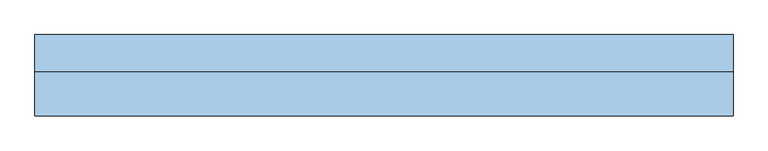
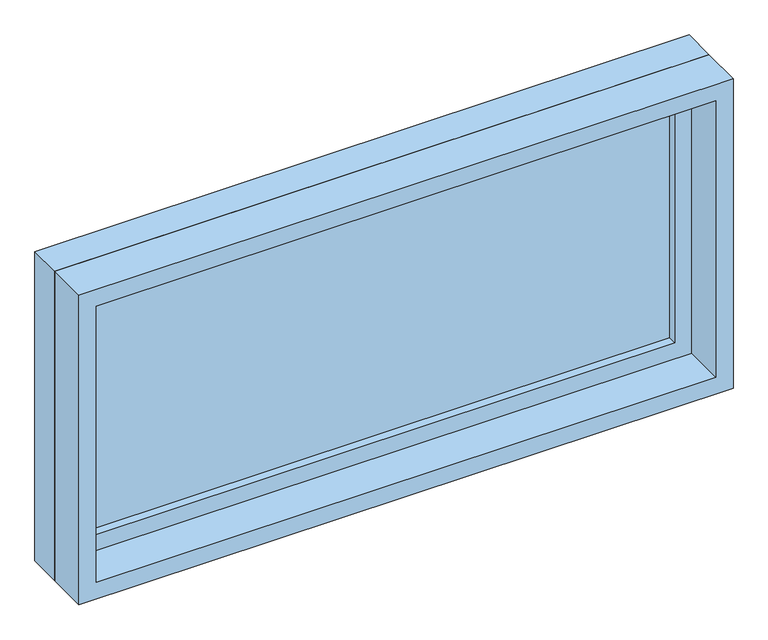
"""IFC4 building model written with IfcOpenShell, lengths in millimetres: window geometry, Фиксированные : 1200х600."""

import ifcopenshell
import ifcopenshell.guid

model = None  # the IFC model being written
_history = None  # IfcOwnerHistory: only IFC2X3 demands one
_inside = {}  # id of a spatial element -> (the spatial element, [elements in it])
_under = {}  # id of a project, library or spatial element -> (it, [spatial elements below it])
_declared = {}  # id of a project -> (the project, [libraries it declares])
_typed = {}  # id of a type object -> (the type object, [elements of that type])
_made_of = {}  # id of a material, layer set ... -> (it, [elements and type objects made of it])


def new_model(schema):
    """Start an empty IFC model of exactly this schema.

    Asked for "IFC4X3", IfcOpenShell would pick the latest addendum, in which some entities
    have other attributes; the version numbers below select the first issue.
    IFC2X3 requires an IfcOwnerHistory on every rooted entity: one is made here for all.
    """
    global model, _history
    if schema == "IFC4X3":
        model = ifcopenshell.file(schema_version=(4, 3, 0, 0))
    else:
        model = ifcopenshell.file(schema=schema)
    _inside.clear()
    _under.clear()
    _declared.clear()
    _typed.clear()
    _made_of.clear()
    _history = None
    if model.schema == "IFC2X3":
        org = make("IfcOrganization", Name="unknown")
        user = make(
            "IfcPersonAndOrganization",
            ThePerson=make("IfcPerson", FamilyName="unknown"),
            TheOrganization=org,
        )
        app = make(
            "IfcApplication",
            ApplicationDeveloper=org,
            Version="unknown",
            ApplicationFullName="unknown",
            ApplicationIdentifier="unknown",
        )
        _history = make(
            "IfcOwnerHistory",
            OwningUser=user,
            OwningApplication=app,
            ChangeAction="ADDED",
            CreationDate=0,
        )
    return model


def make(cls, **values):
    """One entity of the class cls with the attributes given. An attribute that is None is left unset."""
    return model.create_entity(
        cls, **{name: value for name, value in values.items() if value is not None}
    )


def rooted(cls, **values):
    """An entity with a GlobalId (a new one), such as an element, a storey or a relation."""
    return make(cls, GlobalId=ifcopenshell.guid.new(), OwnerHistory=_history, **values)


def si_unit(unit_type, name, prefix=None):
    """IfcSIUnit, for example si_unit("LENGTHUNIT", "METRE", prefix="MILLI")."""
    return make("IfcSIUnit", UnitType=unit_type, Prefix=prefix, Name=name)


def assignment(units):
    """IfcUnitAssignment: the units of a project."""
    return None if units is None else make("IfcUnitAssignment", Units=units)


def point(xyz):
    """IfcCartesianPoint."""
    return None if xyz is None else make("IfcCartesianPoint", Coordinates=xyz)


def direction(xyz):
    """IfcDirection."""
    return None if xyz is None else make("IfcDirection", DirectionRatios=xyz)


def frame(location, z_axis=None, x_axis=None):
    """IfcAxis2Placement3D, a coordinate frame: its origin and axes. An axis left out is left unset."""
    return make(
        "IfcAxis2Placement3D",
        Location=point(location),
        Axis=direction(z_axis),
        RefDirection=direction(x_axis),
    )


def origin():
    """The frame at (0, 0, 0) with its axes left unset."""
    return frame((0.0, 0.0, 0.0))


def place(relative_to, where):
    """IfcLocalPlacement: puts the frame where relative to a parent placement (None: the world)."""
    return make(
        "IfcLocalPlacement", PlacementRelTo=relative_to, RelativePlacement=where
    )


def context(
    kind, dimensions, precision=None, world=None, true_north=None, identifier=None
):
    """IfcGeometricRepresentationContext, for example the 3D "Model" context."""
    return make(
        "IfcGeometricRepresentationContext",
        ContextIdentifier=identifier,
        ContextType=kind,
        CoordinateSpaceDimension=dimensions,
        Precision=precision,
        WorldCoordinateSystem=world,
        TrueNorth=true_north,
    )


def project(units=None, contexts=None):
    """IfcProject with its units and contexts."""
    return rooted(
        "IfcProject",
        Name="project",
        RepresentationContexts=contexts,
        UnitsInContext=assignment(units),
    )


def spatial(cls, under=None, at=None, **own):
    """A site, building, storey or space (cls), placed at a placement, below another one or the project."""
    s = rooted(cls, ObjectPlacement=at, **own)
    if under is not None:
        _under.setdefault(under.id(), (under, []))[1].append(s)
    return s


def polyline(points):
    """IfcPolyline through the points."""
    return make("IfcPolyline", Points=[point(p) for p in points])


def outline(outer, holes=None, kind="AREA"):
    """IfcArbitraryClosedProfileDef: a profile drawn as a closed curve; with holes, ...WithVoids."""
    if holes is None:
        return make("IfcArbitraryClosedProfileDef", ProfileType=kind, OuterCurve=outer)
    return make(
        "IfcArbitraryProfileDefWithVoids",
        ProfileType=kind,
        OuterCurve=outer,
        InnerCurves=holes,
    )


def extrude(swept, where, along, depth):
    """IfcExtrudedAreaSolid: the profile swept, set in the frame where, extruded along a direction by depth."""
    return make(
        "IfcExtrudedAreaSolid",
        SweptArea=swept,
        Position=where,
        ExtrudedDirection=direction(along),
        Depth=depth,
    )


def shape(context_of_items, identifier, shape_type, items):
    """IfcShapeRepresentation: the items that make up one representation, for example the "Body"."""
    return make(
        "IfcShapeRepresentation",
        ContextOfItems=context_of_items,
        RepresentationIdentifier=identifier,
        RepresentationType=shape_type,
        Items=items,
    )


def source(mapping_origin, context_of_items, identifier, shape_type, items):
    """IfcRepresentationMap: a shape defined once, which mapped items show again and again."""
    return make(
        "IfcRepresentationMap",
        MappingOrigin=mapping_origin,
        MappedRepresentation=shape(context_of_items, identifier, shape_type, items),
    )


def transform(
    local_origin,
    x_axis=None,
    y_axis=None,
    z_axis=None,
    scale=None,
    scale2=None,
    scale3=None,
    uniform=True,
):
    """IfcCartesianTransformationOperator3D, or its non-uniform kind. x_axis, y_axis, z_axis: its Axis1, 2, 3."""
    if uniform:
        return make(
            "IfcCartesianTransformationOperator3D",
            Axis1=direction(x_axis),
            Axis2=direction(y_axis),
            LocalOrigin=point(local_origin),
            Scale=scale,
            Axis3=direction(z_axis),
        )
    return make(
        "IfcCartesianTransformationOperator3DnonUniform",
        Axis1=direction(x_axis),
        Axis2=direction(y_axis),
        LocalOrigin=point(local_origin),
        Scale=scale,
        Axis3=direction(z_axis),
        Scale2=scale2,
        Scale3=scale3,
    )


def mapped(mapping_source, mapping_target):
    """IfcMappedItem: shows the shape of a source again, moved by a transform."""
    return make(
        "IfcMappedItem", MappingSource=mapping_source, MappingTarget=mapping_target
    )


def made_of(thing, what):
    """Note that an element or type object is made of a material, layer set ...; save() writes the relation."""
    if what is not None:
        _made_of.setdefault(what.id(), (what, []))[1].append(thing)
    return thing


def element(
    cls,
    number,
    at=None,
    inside=None,
    cuts=None,
    type_object=None,
    material=None,
    context=None,
    identifier="Body",
    shape_type=None,
    held_by="IfcProductDefinitionShape",
    body=None,
    shapes=None,
    **own,
):
    """One element of the class cls, such as IfcWall. Its Tag is "e" and its number.

    at: its placement. inside: the storey or other place that contains it. cuts: it is an
    opening in that element (IfcRelVoidsElement). A single representation is given by context,
    identifier, shape_type and body (its items); several are given by shapes. held_by: the class
    of the entity that holds the representations. save() writes the other relations.
    """
    e = rooted(cls, Tag="e%d" % number, ObjectPlacement=at, **own)
    if body is not None:
        shapes = [shape(context, identifier, shape_type, body)]
    if shapes is not None:
        e.Representation = make(held_by, Representations=shapes)
    if inside is not None:
        _inside.setdefault(inside.id(), (inside, []))[1].append(e)
    if cuts is not None:
        rooted(
            "IfcRelVoidsElement", RelatingBuildingElement=cuts, RelatedOpeningElement=e
        )
    if type_object is not None:
        _typed.setdefault(type_object.id(), (type_object, []))[1].append(e)
    return made_of(e, material)


def aggregate(whole, parts):
    """IfcRelAggregates: a whole, such as a stair, and the parts it consists of."""
    return rooted("IfcRelAggregates", RelatingObject=whole, RelatedObjects=parts)


def save(model, path):
    """Write the relations noted so far, then the file.

    IfcRelAggregates (storeys below a building ...), IfcRelContainedInSpatialStructure (elements
    in a storey), IfcRelDefinesByType, IfcRelAssociatesMaterial and IfcRelDeclares: one each for
    every whole, place, type object, material and project.
    """
    for whole, parts in _under.values():
        aggregate(whole, parts)
    for where, things in _inside.values():
        rooted(
            "IfcRelContainedInSpatialStructure",
            RelatedElements=things,
            RelatingStructure=where,
        )
    for kind, things in _typed.values():
        rooted("IfcRelDefinesByType", RelatedObjects=things, RelatingType=kind)
    for what, things in _made_of.values():
        rooted("IfcRelAssociatesMaterial", RelatedObjects=things, RelatingMaterial=what)
    for by, libraries in _declared.values():
        rooted("IfcRelDeclares", RelatingContext=by, RelatedDefinitions=libraries)
    model.write(path)


def window_76e8b9e6(model_context):
    return source(origin(), model_context, "Body", "SweptSolid", [
        extrude(outline(polyline([(-537.0, 48.0), (537.0, 48.0), (537.0, 36.0), (-537.0, 36.0), (-537.0, 48.0)])), frame((0.0, 0.0, 978.0), z_axis=(0.0, 0.0, 1.0), x_axis=(1.0, 0.0, 0.0)), (0.0, 0.0, 1.0), 474.0),
        extrude(outline(polyline([(1496.0, -581.0), (934.0, -581.0), (934.0, 581.0), (1496.0, 581.0), (1496.0, -581.0)]), holes=[polyline([(1452.0, -537.0), (1452.0, 537.0), (978.0, 537.0), (978.0, -537.0), (1452.0, -537.0)])]), frame((0.0, 20.0, 0.0), z_axis=(0.0, 1.0, 0.0), x_axis=(0.0, 0.0, 1.0)), (0.0, 0.0, 1.0), 44.0),
        extrude(outline(polyline([(1515.0, -600.0), (915.0, -600.0), (915.0, 600.0), (1515.0, 600.0), (1515.0, -600.0)]), holes=[polyline([(1496.0, -581.0), (1496.0, 581.0), (934.0, 581.0), (934.0, -581.0), (1496.0, -581.0)])]), frame((0.0, 20.0, 0.0), z_axis=(0.0, 1.0, 0.0), x_axis=(0.0, 0.0, 1.0)), (0.0, 0.0, 1.0), 63.0),
        extrude(outline(polyline([(1515.0, -600.0), (915.0, -600.0), (915.0, 600.0), (1515.0, 600.0), (1515.0, -600.0)]), holes=[polyline([(1483.0, -568.0), (1483.0, 568.0), (947.0, 568.0), (947.0, -568.0), (1483.0, -568.0)])]), frame((0.0, -57.0, 0.0), z_axis=(0.0, 1.0, 0.0), x_axis=(0.0, 0.0, 1.0)), (0.0, 0.0, 1.0), 77.0),
    ])


if __name__ == "__main__":
    model = new_model("IFC4")
    model_context = context("Model", 3, world=origin())
    ifc_project = project(units=[si_unit("LENGTHUNIT", "METRE", prefix="MILLI")], contexts=[model_context])
    site = spatial("IfcSite", under=ifc_project)
    building = spatial("IfcBuilding", under=site)
    placement = place(None, origin())
    window_shape = window_76e8b9e6(model_context)
    element("IfcWindow", 1, ObjectType="Фиксированные : 1200х600", at=placement, inside=building, context=model_context, shape_type="MappedRepresentation", body=[
        mapped(window_shape, transform((0.0, 0.0, 0.0), x_axis=(1.0, 0.0, 0.0), y_axis=(0.0, 1.0, 0.0), z_axis=(0.0, 0.0, 1.0))),
    ])
    save(model, "model.ifc")

# Revit data of these elements
# Type "Фиксированные : 1200х600"
#   Type Mark = "19"
#   Construction Type Id = "GSP4R"
#   Analytic Construction = "Одинарное остекление стеклами Пилкингтон - 1/8 дюйма"
#   Visual Light Transmittance = 0.9
#   Solar Heat Gain Coefficient = 0.78
#   Heat Transfer Coefficient (U) = 3.6886 W/(m²·K)
#   Height = 600 mm
#   Высота подоконника по умолчанию = 915 mm
#   Width = 1200 mm
#   Вставка окна = 19 mm
#   Наружный материал каркаса = Переплет
#   Внутренний материал каркаса = Переплет
#   Материал оконного стекла = Стекло
#   Переплет = Переплет
#   Wall Closure = (empty or 0)
# Element 1 (IfcWindow, "Фиксированные : 1200х600")
#   Materials on its faces: "Переплет", "Стекло"
# Materials
#   "Переплет": class "Древесина", colour RGB 224 178 126, transparency 0, Cost = 0
#   "Стекло": class "Стекло", colour RGB 0 128 192, transparency 0.9, Description = "Известково-натриевое стекло", Cost = 0
